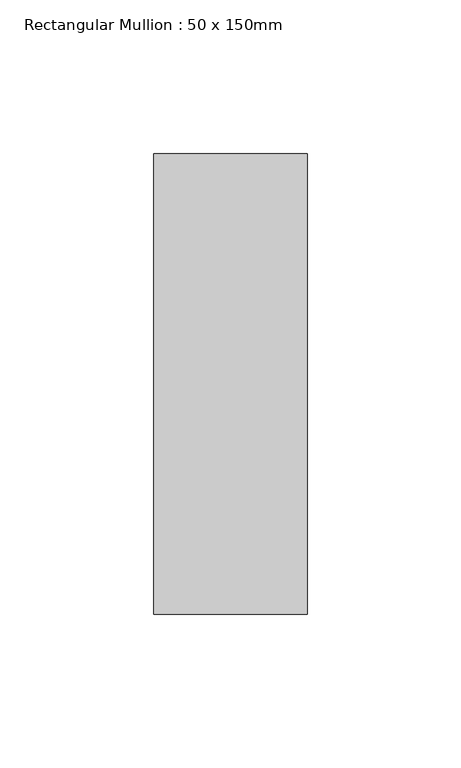
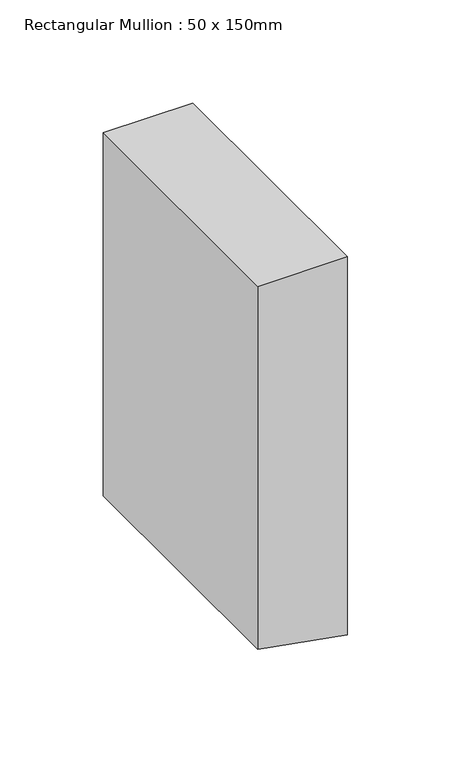
"""IFC4 building model written with IfcOpenShell, lengths in millimetres: member geometry, Rectangular Mullion : 50 x 150mm."""

import ifcopenshell
import ifcopenshell.guid

model = None  # the IFC model being written
_history = None  # IfcOwnerHistory: only IFC2X3 demands one
_inside = {}  # id of a spatial element -> (the spatial element, [elements in it])
_under = {}  # id of a project, library or spatial element -> (it, [spatial elements below it])
_declared = {}  # id of a project -> (the project, [libraries it declares])
_typed = {}  # id of a type object -> (the type object, [elements of that type])
_made_of = {}  # id of a material, layer set ... -> (it, [elements and type objects made of it])


def new_model(schema):
    """Start an empty IFC model of exactly this schema.

    Asked for "IFC4X3", IfcOpenShell would pick the latest addendum, in which some entities
    have other attributes; the version numbers below select the first issue.
    IFC2X3 requires an IfcOwnerHistory on every rooted entity: one is made here for all.
    """
    global model, _history
    if schema == "IFC4X3":
        model = ifcopenshell.file(schema_version=(4, 3, 0, 0))
    else:
        model = ifcopenshell.file(schema=schema)
    _inside.clear()
    _under.clear()
    _declared.clear()
    _typed.clear()
    _made_of.clear()
    _history = None
    if model.schema == "IFC2X3":
        org = make("IfcOrganization", Name="unknown")
        user = make(
            "IfcPersonAndOrganization",
            ThePerson=make("IfcPerson", FamilyName="unknown"),
            TheOrganization=org,
        )
        app = make(
            "IfcApplication",
            ApplicationDeveloper=org,
            Version="unknown",
            ApplicationFullName="unknown",
            ApplicationIdentifier="unknown",
        )
        _history = make(
            "IfcOwnerHistory",
            OwningUser=user,
            OwningApplication=app,
            ChangeAction="ADDED",
            CreationDate=0,
        )
    return model


def make(cls, **values):
    """One entity of the class cls with the attributes given. An attribute that is None is left unset."""
    return model.create_entity(
        cls, **{name: value for name, value in values.items() if value is not None}
    )


def rooted(cls, **values):
    """An entity with a GlobalId (a new one), such as an element, a storey or a relation."""
    return make(cls, GlobalId=ifcopenshell.guid.new(), OwnerHistory=_history, **values)


def si_unit(unit_type, name, prefix=None):
    """IfcSIUnit, for example si_unit("LENGTHUNIT", "METRE", prefix="MILLI")."""
    return make("IfcSIUnit", UnitType=unit_type, Prefix=prefix, Name=name)


def assignment(units):
    """IfcUnitAssignment: the units of a project."""
    return None if units is None else make("IfcUnitAssignment", Units=units)


def point(xyz):
    """IfcCartesianPoint."""
    return None if xyz is None else make("IfcCartesianPoint", Coordinates=xyz)


def direction(xyz):
    """IfcDirection."""
    return None if xyz is None else make("IfcDirection", DirectionRatios=xyz)


def frame(location, z_axis=None, x_axis=None):
    """IfcAxis2Placement3D, a coordinate frame: its origin and axes. An axis left out is left unset."""
    return make(
        "IfcAxis2Placement3D",
        Location=point(location),
        Axis=direction(z_axis),
        RefDirection=direction(x_axis),
    )


def origin():
    """The frame at (0, 0, 0) with its axes left unset."""
    return frame((0.0, 0.0, 0.0))


def place(relative_to, where):
    """IfcLocalPlacement: puts the frame where relative to a parent placement (None: the world)."""
    return make(
        "IfcLocalPlacement", PlacementRelTo=relative_to, RelativePlacement=where
    )


def context(
    kind, dimensions, precision=None, world=None, true_north=None, identifier=None
):
    """IfcGeometricRepresentationContext, for example the 3D "Model" context."""
    return make(
        "IfcGeometricRepresentationContext",
        ContextIdentifier=identifier,
        ContextType=kind,
        CoordinateSpaceDimension=dimensions,
        Precision=precision,
        WorldCoordinateSystem=world,
        TrueNorth=true_north,
    )


def project(units=None, contexts=None):
    """IfcProject with its units and contexts."""
    return rooted(
        "IfcProject",
        Name="project",
        RepresentationContexts=contexts,
        UnitsInContext=assignment(units),
    )


def spatial(cls, under=None, at=None, **own):
    """A site, building, storey or space (cls), placed at a placement, below another one or the project."""
    s = rooted(cls, ObjectPlacement=at, **own)
    if under is not None:
        _under.setdefault(under.id(), (under, []))[1].append(s)
    return s


def polyline(points):
    """IfcPolyline through the points."""
    return make("IfcPolyline", Points=[point(p) for p in points])


def outline(outer, holes=None, kind="AREA"):
    """IfcArbitraryClosedProfileDef: a profile drawn as a closed curve; with holes, ...WithVoids."""
    if holes is None:
        return make("IfcArbitraryClosedProfileDef", ProfileType=kind, OuterCurve=outer)
    return make(
        "IfcArbitraryProfileDefWithVoids",
        ProfileType=kind,
        OuterCurve=outer,
        InnerCurves=holes,
    )


def extrude(swept, where, along, depth):
    """IfcExtrudedAreaSolid: the profile swept, set in the frame where, extruded along a direction by depth."""
    return make(
        "IfcExtrudedAreaSolid",
        SweptArea=swept,
        Position=where,
        ExtrudedDirection=direction(along),
        Depth=depth,
    )


def shape(context_of_items, identifier, shape_type, items):
    """IfcShapeRepresentation: the items that make up one representation, for example the "Body"."""
    return make(
        "IfcShapeRepresentation",
        ContextOfItems=context_of_items,
        RepresentationIdentifier=identifier,
        RepresentationType=shape_type,
        Items=items,
    )


def source(mapping_origin, context_of_items, identifier, shape_type, items):
    """IfcRepresentationMap: a shape defined once, which mapped items show again and again."""
    return make(
        "IfcRepresentationMap",
        MappingOrigin=mapping_origin,
        MappedRepresentation=shape(context_of_items, identifier, shape_type, items),
    )


def transform(
    local_origin,
    x_axis=None,
    y_axis=None,
    z_axis=None,
    scale=None,
    scale2=None,
    scale3=None,
    uniform=True,
):
    """IfcCartesianTransformationOperator3D, or its non-uniform kind. x_axis, y_axis, z_axis: its Axis1, 2, 3."""
    if uniform:
        return make(
            "IfcCartesianTransformationOperator3D",
            Axis1=direction(x_axis),
            Axis2=direction(y_axis),
            LocalOrigin=point(local_origin),
            Scale=scale,
            Axis3=direction(z_axis),
        )
    return make(
        "IfcCartesianTransformationOperator3DnonUniform",
        Axis1=direction(x_axis),
        Axis2=direction(y_axis),
        LocalOrigin=point(local_origin),
        Scale=scale,
        Axis3=direction(z_axis),
        Scale2=scale2,
        Scale3=scale3,
    )


def mapped(mapping_source, mapping_target):
    """IfcMappedItem: shows the shape of a source again, moved by a transform."""
    return make(
        "IfcMappedItem", MappingSource=mapping_source, MappingTarget=mapping_target
    )


def made_of(thing, what):
    """Note that an element or type object is made of a material, layer set ...; save() writes the relation."""
    if what is not None:
        _made_of.setdefault(what.id(), (what, []))[1].append(thing)
    return thing


def element(
    cls,
    number,
    at=None,
    inside=None,
    cuts=None,
    type_object=None,
    material=None,
    context=None,
    identifier="Body",
    shape_type=None,
    held_by="IfcProductDefinitionShape",
    body=None,
    shapes=None,
    **own,
):
    """One element of the class cls, such as IfcWall. Its Tag is "e" and its number.

    at: its placement. inside: the storey or other place that contains it. cuts: it is an
    opening in that element (IfcRelVoidsElement). A single representation is given by context,
    identifier, shape_type and body (its items); several are given by shapes. held_by: the class
    of the entity that holds the representations. save() writes the other relations.
    """
    e = rooted(cls, Tag="e%d" % number, ObjectPlacement=at, **own)
    if body is not None:
        shapes = [shape(context, identifier, shape_type, body)]
    if shapes is not None:
        e.Representation = make(held_by, Representations=shapes)
    if inside is not None:
        _inside.setdefault(inside.id(), (inside, []))[1].append(e)
    if cuts is not None:
        rooted(
            "IfcRelVoidsElement", RelatingBuildingElement=cuts, RelatedOpeningElement=e
        )
    if type_object is not None:
        _typed.setdefault(type_object.id(), (type_object, []))[1].append(e)
    return made_of(e, material)


def aggregate(whole, parts):
    """IfcRelAggregates: a whole, such as a stair, and the parts it consists of."""
    return rooted("IfcRelAggregates", RelatingObject=whole, RelatedObjects=parts)


def save(model, path):
    """Write the relations noted so far, then the file.

    IfcRelAggregates (storeys below a building ...), IfcRelContainedInSpatialStructure (elements
    in a storey), IfcRelDefinesByType, IfcRelAssociatesMaterial and IfcRelDeclares: one each for
    every whole, place, type object, material and project.
    """
    for whole, parts in _under.values():
        aggregate(whole, parts)
    for where, things in _inside.values():
        rooted(
            "IfcRelContainedInSpatialStructure",
            RelatedElements=things,
            RelatingStructure=where,
        )
    for kind, things in _typed.values():
        rooted("IfcRelDefinesByType", RelatedObjects=things, RelatingType=kind)
    for what, things in _made_of.values():
        rooted("IfcRelAssociatesMaterial", RelatedObjects=things, RelatingMaterial=what)
    for by, libraries in _declared.values():
        rooted("IfcRelDeclares", RelatingContext=by, RelatedDefinitions=libraries)
    model.write(path)


def rectangular_mullion_50_x_150mm_e37662f2(model_context):
    return source(origin(), model_context, "Body", "SweptSolid", [
        extrude(outline(polyline([(0.0, 25.0), (0.0, -25.0), (-214.8982375, -25.0), (-220.0718835, 4.3412044), (-223.7145866, 25.0), (0.0, 25.0)])), frame((0.0, -75.0, 0.0), z_axis=(0.0, 1.0, 0.0), x_axis=(0.0, 0.0, 1.0)), (0.0, 0.0, 1.0), 150.0),
    ])


if __name__ == "__main__":
    model = new_model("IFC4")
    model_context = context("Model", 3, world=origin())
    ifc_project = project(units=[si_unit("LENGTHUNIT", "METRE", prefix="MILLI")], contexts=[model_context])
    site = spatial("IfcSite", under=ifc_project)
    building = spatial("IfcBuilding", under=site)
    placement = place(None, origin())
    rectangular_mullion_50_x_150mm_shape = rectangular_mullion_50_x_150mm_e37662f2(model_context)
    element("IfcMember", 1, ObjectType="Rectangular Mullion : 50 x 150mm", at=placement, inside=building, context=model_context, shape_type="MappedRepresentation", body=[
        mapped(rectangular_mullion_50_x_150mm_shape, transform((0.0, 0.0, 0.0), x_axis=(1.0, 0.0, 0.0), y_axis=(0.0, 1.0, 0.0), z_axis=(0.0, 0.0, 1.0))),
    ])
    save(model, "model.ifc")

# Revit data of these elements
# Type "Rectangular Mullion : 50 x 150mm"
#   built-in parameter 1007304 = 0.492126 (stored number, unit not read)
#   built-in parameter 1007301 = 0.082021 (stored number, unit not read)
#   built-in parameter 1007300 = 0.082021 (stored number, unit not read)
# Element 1 (IfcMember, "Rectangular Mullion : 50 x 150mm")
#   Materials on its faces: "Aluminium"
# Materials
#   "Aluminium": class "Metal", colour RGB 247 247 247, transparency 0, Description = "Aluminium 6061", Cost = 0
